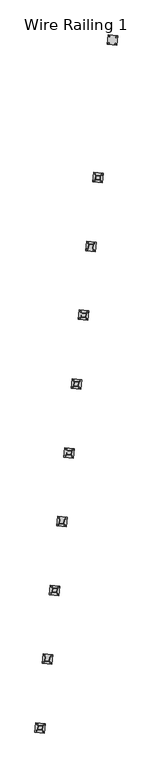
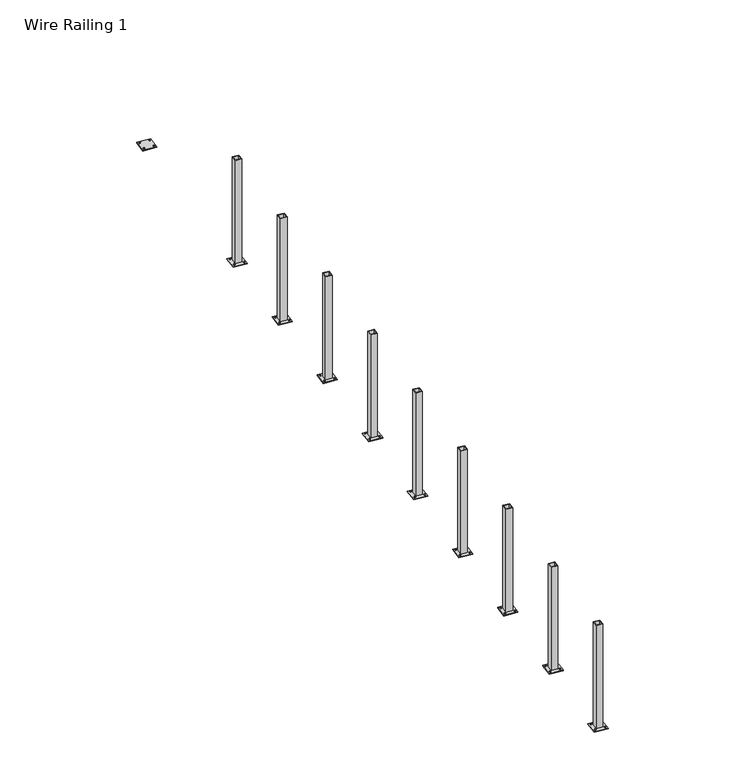
"""IFC4 building model written with IfcOpenShell, lengths in millimetres: railing geometry, Wire Railing 1."""

from ifc_helpers import new_model, si_unit, point, frame, frame_2d, origin, place, context, project, spatial, polyline, circle_curve, trimmed, segment, composite_curve, outline, extrude, source, transform, mapped, element, save


def wire_railing_1_54126149(model_context):
    return source(origin(), model_context, "Body", "SweptSolid", [
        extrude(outline(composite_curve([segment(trimmed(circle_curve(frame_2d((35087.2651438, 39002.031004)), 6.35), [point((35080.9499297, 39002.6947597))], [point((35093.5803578, 39001.3672483))], False, "CARTESIAN"), True, "CONTINUOUS"), segment(trimmed(circle_curve(frame_2d((35087.2651438, 39002.031004)), 6.35), [point((35093.5803578, 39001.3672483))], [point((35080.9499297, 39002.6947597))], False, "CARTESIAN"), True, "CONTINUOUS")], self_intersect=False)), frame((0.0, 0.0, 269252.7), z_axis=(0.0, 0.0, 1.0), x_axis=(1.0, 0.0, 0.0)), (0.0, 0.0, 1.0), 12.7),
        extrude(outline(composite_curve([segment(trimmed(circle_curve(frame_2d((35175.6781403, 38992.7384236)), 6.35), [point((35169.3629262, 38993.4021794))], [point((35181.9933543, 38992.0746679))], False, "CARTESIAN"), True, "CONTINUOUS"), segment(trimmed(circle_curve(frame_2d((35175.6781403, 38992.7384236)), 6.35), [point((35181.9933543, 38992.0746679))], [point((35169.3629262, 38993.4021794))], False, "CARTESIAN"), True, "CONTINUOUS")], self_intersect=False)), frame((0.0, 0.0, 269252.7), z_axis=(0.0, 0.0, 1.0), x_axis=(1.0, 0.0, 0.0)), (0.0, 0.0, 1.0), 12.7),
        extrude(outline(composite_curve([segment(trimmed(circle_curve(frame_2d((35096.5577242, 39090.4440005)), 6.35), [point((35090.2425101, 39091.1077562))], [point((35102.8729382, 39089.7802448))], False, "CARTESIAN"), True, "CONTINUOUS"), segment(trimmed(circle_curve(frame_2d((35096.5577242, 39090.4440005)), 6.35), [point((35102.8729382, 39089.7802448))], [point((35090.2425101, 39091.1077562))], False, "CARTESIAN"), True, "CONTINUOUS")], self_intersect=False)), frame((0.0, 0.0, 269252.7), z_axis=(0.0, 0.0, 1.0), x_axis=(1.0, 0.0, 0.0)), (0.0, 0.0, 1.0), 12.7),
        extrude(outline(composite_curve([segment(trimmed(circle_curve(frame_2d((35184.9707207, 39081.1514201)), 6.35), [point((35178.6555066, 39081.8151759))], [point((35191.2859347, 39080.4876644))], False, "CARTESIAN"), True, "CONTINUOUS"), segment(trimmed(circle_curve(frame_2d((35184.9707207, 39081.1514201)), 6.35), [point((35191.2859347, 39080.4876644))], [point((35178.6555066, 39081.8151759))], False, "CARTESIAN"), True, "CONTINUOUS")], self_intersect=False)), frame((0.0, 0.0, 269252.7), z_axis=(0.0, 0.0, 1.0), x_axis=(1.0, 0.0, 0.0)), (0.0, 0.0, 1.0), 12.7),
        extrude(outline(polyline([(35192.6325152, 38971.8015143), (35066.3282344, 38985.0766291), (35079.6033493, 39111.3809098), (35205.90763, 39098.105795), (35192.6325152, 38971.8015143)])), frame((0.0, 0.0, 269252.7), z_axis=(0.0, 0.0, 1.0), x_axis=(1.0, 0.0, 0.0)), (0.0, 0.0, 1.0), 6.35),
        extrude(outline(polyline([(35162.9623591, 39008.4411056), (35102.9678258, 39014.7467852), (35109.2735053, 39074.7413185), (35169.2680387, 39068.4356389), (35162.9623591, 39008.4411056)]), holes=[polyline([(35157.3109008, 39015.4200754), (35162.2890689, 39062.7841807), (35114.9249636, 39067.7623487), (35109.9467956, 39020.3982435), (35157.3109008, 39015.4200754)])]), frame((0.0, 0.0, 269252.7), z_axis=(0.0, 0.0, 1.0), x_axis=(1.0, 0.0, 0.0)), (0.0, 0.0, 1.0), 1047.75),
        extrude(outline(composite_curve([segment(trimmed(circle_curve(frame_2d((34991.3177498, 38089.1525294)), 6.35), [point((34985.0025358, 38089.8162852))], [point((34997.6329638, 38088.4887737))], False, "CARTESIAN"), True, "CONTINUOUS"), segment(trimmed(circle_curve(frame_2d((34991.3177498, 38089.1525294)), 6.35), [point((34997.6329638, 38088.4887737))], [point((34985.0025358, 38089.8162852))], False, "CARTESIAN"), True, "CONTINUOUS")], self_intersect=False)), frame((0.0, 0.0, 269252.7), z_axis=(0.0, 0.0, 1.0), x_axis=(1.0, 0.0, 0.0)), (0.0, 0.0, 1.0), 12.7),
        extrude(outline(composite_curve([segment(trimmed(circle_curve(frame_2d((35079.7307463, 38079.859949)), 6.35), [point((35073.4155323, 38080.5237048))], [point((35086.0459603, 38079.1961933))], False, "CARTESIAN"), True, "CONTINUOUS"), segment(trimmed(circle_curve(frame_2d((35079.7307463, 38079.859949)), 6.35), [point((35086.0459603, 38079.1961933))], [point((35073.4155323, 38080.5237048))], False, "CARTESIAN"), True, "CONTINUOUS")], self_intersect=False)), frame((0.0, 0.0, 269252.7), z_axis=(0.0, 0.0, 1.0), x_axis=(1.0, 0.0, 0.0)), (0.0, 0.0, 1.0), 12.7),
        extrude(outline(composite_curve([segment(trimmed(circle_curve(frame_2d((35000.6103302, 38177.5655259)), 6.35), [point((34994.2951162, 38178.2292817))], [point((35006.9255442, 38176.9017702))], False, "CARTESIAN"), True, "CONTINUOUS"), segment(trimmed(circle_curve(frame_2d((35000.6103302, 38177.5655259)), 6.35), [point((35006.9255442, 38176.9017702))], [point((34994.2951162, 38178.2292817))], False, "CARTESIAN"), True, "CONTINUOUS")], self_intersect=False)), frame((0.0, 0.0, 269252.7), z_axis=(0.0, 0.0, 1.0), x_axis=(1.0, 0.0, 0.0)), (0.0, 0.0, 1.0), 12.7),
        extrude(outline(composite_curve([segment(trimmed(circle_curve(frame_2d((35089.0233267, 38168.2729455)), 6.35), [point((35082.7081127, 38168.9367013))], [point((35095.3385407, 38167.6091898))], False, "CARTESIAN"), True, "CONTINUOUS"), segment(trimmed(circle_curve(frame_2d((35089.0233267, 38168.2729455)), 6.35), [point((35095.3385407, 38167.6091898))], [point((35082.7081127, 38168.9367013))], False, "CARTESIAN"), True, "CONTINUOUS")], self_intersect=False)), frame((0.0, 0.0, 269252.7), z_axis=(0.0, 0.0, 1.0), x_axis=(1.0, 0.0, 0.0)), (0.0, 0.0, 1.0), 12.7),
        extrude(outline(polyline([(35096.6851212, 38058.9230397), (34970.3808405, 38072.1981545), (34983.6559553, 38198.5024353), (35109.960236, 38185.2273204), (35096.6851212, 38058.9230397)])), frame((0.0, 0.0, 269252.7), z_axis=(0.0, 0.0, 1.0), x_axis=(1.0, 0.0, 0.0)), (0.0, 0.0, 1.0), 6.35),
        extrude(outline(polyline([(35067.0149652, 38095.562631), (35007.0204318, 38101.8683106), (35013.3261114, 38161.8628439), (35073.3206447, 38155.5571644), (35067.0149652, 38095.562631)]), holes=[polyline([(35061.3635069, 38102.5416008), (35066.3416749, 38149.9057061), (35018.9775697, 38154.8838741), (35013.9994016, 38107.5197689), (35061.3635069, 38102.5416008)])]), frame((0.0, 0.0, 269252.7), z_axis=(0.0, 0.0, 1.0), x_axis=(1.0, 0.0, 0.0)), (0.0, 0.0, 1.0), 1047.75),
        extrude(outline(composite_curve([segment(trimmed(circle_curve(frame_2d((34895.3703559, 37176.2740549)), 6.35), [point((34889.0551418, 37176.9378106))], [point((34901.6855699, 37175.6102991))], False, "CARTESIAN"), True, "CONTINUOUS"), segment(trimmed(circle_curve(frame_2d((34895.3703559, 37176.2740549)), 6.35), [point((34901.6855699, 37175.6102991))], [point((34889.0551418, 37176.9378106))], False, "CARTESIAN"), True, "CONTINUOUS")], self_intersect=False)), frame((0.0, 0.0, 269252.7), z_axis=(0.0, 0.0, 1.0), x_axis=(1.0, 0.0, 0.0)), (0.0, 0.0, 1.0), 12.7),
        extrude(outline(composite_curve([segment(trimmed(circle_curve(frame_2d((34983.7833524, 37166.9814745)), 6.35), [point((34977.4681383, 37167.6452302))], [point((34990.0985664, 37166.3177187))], False, "CARTESIAN"), True, "CONTINUOUS"), segment(trimmed(circle_curve(frame_2d((34983.7833524, 37166.9814745)), 6.35), [point((34990.0985664, 37166.3177187))], [point((34977.4681383, 37167.6452302))], False, "CARTESIAN"), True, "CONTINUOUS")], self_intersect=False)), frame((0.0, 0.0, 269252.7), z_axis=(0.0, 0.0, 1.0), x_axis=(1.0, 0.0, 0.0)), (0.0, 0.0, 1.0), 12.7),
        extrude(outline(composite_curve([segment(trimmed(circle_curve(frame_2d((34904.6629362, 37264.6870513)), 6.35), [point((34898.3477222, 37265.3508071))], [point((34910.9781503, 37264.0232956))], False, "CARTESIAN"), True, "CONTINUOUS"), segment(trimmed(circle_curve(frame_2d((34904.6629362, 37264.6870513)), 6.35), [point((34910.9781503, 37264.0232956))], [point((34898.3477222, 37265.3508071))], False, "CARTESIAN"), True, "CONTINUOUS")], self_intersect=False)), frame((0.0, 0.0, 269252.7), z_axis=(0.0, 0.0, 1.0), x_axis=(1.0, 0.0, 0.0)), (0.0, 0.0, 1.0), 12.7),
        extrude(outline(composite_curve([segment(trimmed(circle_curve(frame_2d((34993.0759327, 37255.394471)), 6.35), [point((34986.7607187, 37256.0582267))], [point((34999.3911468, 37254.7307152))], False, "CARTESIAN"), True, "CONTINUOUS"), segment(trimmed(circle_curve(frame_2d((34993.0759327, 37255.394471)), 6.35), [point((34999.3911468, 37254.7307152))], [point((34986.7607187, 37256.0582267))], False, "CARTESIAN"), True, "CONTINUOUS")], self_intersect=False)), frame((0.0, 0.0, 269252.7), z_axis=(0.0, 0.0, 1.0), x_axis=(1.0, 0.0, 0.0)), (0.0, 0.0, 1.0), 12.7),
        extrude(outline(polyline([(35000.7377272, 37146.0445651), (34874.4334465, 37159.31968), (34887.7085614, 37285.6239607), (35014.0128421, 37272.3488458), (35000.7377272, 37146.0445651)])), frame((0.0, 0.0, 269252.7), z_axis=(0.0, 0.0, 1.0), x_axis=(1.0, 0.0, 0.0)), (0.0, 0.0, 1.0), 6.35),
        extrude(outline(polyline([(34971.0675712, 37182.6841565), (34911.0730379, 37188.989836), (34917.3787174, 37248.9843694), (34977.3732507, 37242.6786898), (34971.0675712, 37182.6841565)]), holes=[polyline([(34965.4161129, 37189.6631262), (34970.394281, 37237.0272315), (34923.0301757, 37242.0053996), (34918.0520076, 37194.6412943), (34965.4161129, 37189.6631262)])]), frame((0.0, 0.0, 269252.7), z_axis=(0.0, 0.0, 1.0), x_axis=(1.0, 0.0, 0.0)), (0.0, 0.0, 1.0), 1047.75),
        extrude(outline(composite_curve([segment(trimmed(circle_curve(frame_2d((34799.4229619, 36263.3955803)), 6.35), [point((34793.1077479, 36264.059336))], [point((34805.7381759, 36262.7318245))], False, "CARTESIAN"), True, "CONTINUOUS"), segment(trimmed(circle_curve(frame_2d((34799.4229619, 36263.3955803)), 6.35), [point((34805.7381759, 36262.7318245))], [point((34793.1077479, 36264.059336))], False, "CARTESIAN"), True, "CONTINUOUS")], self_intersect=False)), frame((0.0, 0.0, 269252.7), z_axis=(0.0, 0.0, 1.0), x_axis=(1.0, 0.0, 0.0)), (0.0, 0.0, 1.0), 12.7),
        extrude(outline(composite_curve([segment(trimmed(circle_curve(frame_2d((34887.8359584, 36254.1029999)), 6.35), [point((34881.5207444, 36254.7667556))], [point((34894.1511724, 36253.4392442))], False, "CARTESIAN"), True, "CONTINUOUS"), segment(trimmed(circle_curve(frame_2d((34887.8359584, 36254.1029999)), 6.35), [point((34894.1511724, 36253.4392442))], [point((34881.5207444, 36254.7667556))], False, "CARTESIAN"), True, "CONTINUOUS")], self_intersect=False)), frame((0.0, 0.0, 269252.7), z_axis=(0.0, 0.0, 1.0), x_axis=(1.0, 0.0, 0.0)), (0.0, 0.0, 1.0), 12.7),
        extrude(outline(composite_curve([segment(trimmed(circle_curve(frame_2d((34808.7155423, 36351.8085768)), 6.35), [point((34802.4003282, 36352.4723325))], [point((34815.0307563, 36351.144821))], False, "CARTESIAN"), True, "CONTINUOUS"), segment(trimmed(circle_curve(frame_2d((34808.7155423, 36351.8085768)), 6.35), [point((34815.0307563, 36351.144821))], [point((34802.4003282, 36352.4723325))], False, "CARTESIAN"), True, "CONTINUOUS")], self_intersect=False)), frame((0.0, 0.0, 269252.7), z_axis=(0.0, 0.0, 1.0), x_axis=(1.0, 0.0, 0.0)), (0.0, 0.0, 1.0), 12.7),
        extrude(outline(composite_curve([segment(trimmed(circle_curve(frame_2d((34897.1285388, 36342.5159964)), 6.35), [point((34890.8133247, 36343.1797521))], [point((34903.4437528, 36341.8522407))], False, "CARTESIAN"), True, "CONTINUOUS"), segment(trimmed(circle_curve(frame_2d((34897.1285388, 36342.5159964)), 6.35), [point((34903.4437528, 36341.8522407))], [point((34890.8133247, 36343.1797521))], False, "CARTESIAN"), True, "CONTINUOUS")], self_intersect=False)), frame((0.0, 0.0, 269252.7), z_axis=(0.0, 0.0, 1.0), x_axis=(1.0, 0.0, 0.0)), (0.0, 0.0, 1.0), 12.7),
        extrude(outline(polyline([(34904.7903333, 36233.1660906), (34778.4860526, 36246.4412054), (34791.7611674, 36372.7454861), (34918.0654481, 36359.4703713), (34904.7903333, 36233.1660906)])), frame((0.0, 0.0, 269252.7), z_axis=(0.0, 0.0, 1.0), x_axis=(1.0, 0.0, 0.0)), (0.0, 0.0, 1.0), 6.35),
        extrude(outline(polyline([(34875.1201772, 36269.8056819), (34815.1256439, 36276.1113614), (34821.4313234, 36336.1058948), (34881.4258568, 36329.8002152), (34875.1201772, 36269.8056819)]), holes=[polyline([(34869.4687189, 36276.7846517), (34874.446887, 36324.1487569), (34827.0827817, 36329.126925), (34822.1046137, 36281.7628197), (34869.4687189, 36276.7846517)])]), frame((0.0, 0.0, 269252.7), z_axis=(0.0, 0.0, 1.0), x_axis=(1.0, 0.0, 0.0)), (0.0, 0.0, 1.0), 1047.75),
        extrude(outline(composite_curve([segment(trimmed(circle_curve(frame_2d((34703.4755679, 35350.5171057)), 6.35), [point((34697.1603539, 35351.1808614))], [point((34709.790782, 35349.85335))], False, "CARTESIAN"), True, "CONTINUOUS"), segment(trimmed(circle_curve(frame_2d((34703.4755679, 35350.5171057)), 6.35), [point((34709.790782, 35349.85335))], [point((34697.1603539, 35351.1808614))], False, "CARTESIAN"), True, "CONTINUOUS")], self_intersect=False)), frame((0.0, 0.0, 269252.7), z_axis=(0.0, 0.0, 1.0), x_axis=(1.0, 0.0, 0.0)), (0.0, 0.0, 1.0), 12.7),
        extrude(outline(composite_curve([segment(trimmed(circle_curve(frame_2d((34791.8885644, 35341.2245253)), 6.35), [point((34785.5733504, 35341.8882811))], [point((34798.2037785, 35340.5607696))], False, "CARTESIAN"), True, "CONTINUOUS"), segment(trimmed(circle_curve(frame_2d((34791.8885644, 35341.2245253)), 6.35), [point((34798.2037785, 35340.5607696))], [point((34785.5733504, 35341.8882811))], False, "CARTESIAN"), True, "CONTINUOUS")], self_intersect=False)), frame((0.0, 0.0, 269252.7), z_axis=(0.0, 0.0, 1.0), x_axis=(1.0, 0.0, 0.0)), (0.0, 0.0, 1.0), 12.7),
        extrude(outline(composite_curve([segment(trimmed(circle_curve(frame_2d((34712.7681483, 35438.9301022)), 6.35), [point((34706.4529343, 35439.5938579))], [point((34719.0833624, 35438.2663465))], False, "CARTESIAN"), True, "CONTINUOUS"), segment(trimmed(circle_curve(frame_2d((34712.7681483, 35438.9301022)), 6.35), [point((34719.0833624, 35438.2663465))], [point((34706.4529343, 35439.5938579))], False, "CARTESIAN"), True, "CONTINUOUS")], self_intersect=False)), frame((0.0, 0.0, 269252.7), z_axis=(0.0, 0.0, 1.0), x_axis=(1.0, 0.0, 0.0)), (0.0, 0.0, 1.0), 12.7),
        extrude(outline(composite_curve([segment(trimmed(circle_curve(frame_2d((34801.1811448, 35429.6375218)), 6.35), [point((34794.8659308, 35430.3012776))], [point((34807.4963589, 35428.9737661))], False, "CARTESIAN"), True, "CONTINUOUS"), segment(trimmed(circle_curve(frame_2d((34801.1811448, 35429.6375218)), 6.35), [point((34807.4963589, 35428.9737661))], [point((34794.8659308, 35430.3012776))], False, "CARTESIAN"), True, "CONTINUOUS")], self_intersect=False)), frame((0.0, 0.0, 269252.7), z_axis=(0.0, 0.0, 1.0), x_axis=(1.0, 0.0, 0.0)), (0.0, 0.0, 1.0), 12.7),
        extrude(outline(polyline([(34808.8429393, 35320.287616), (34682.5386586, 35333.5627308), (34695.8137734, 35459.8670115), (34822.1180541, 35446.5918967), (34808.8429393, 35320.287616)])), frame((0.0, 0.0, 269252.7), z_axis=(0.0, 0.0, 1.0), x_axis=(1.0, 0.0, 0.0)), (0.0, 0.0, 1.0), 6.35),
        extrude(outline(polyline([(34779.1727833, 35356.9272073), (34719.1782499, 35363.2328869), (34725.4839295, 35423.2274202), (34785.4784628, 35416.9217407), (34779.1727833, 35356.9272073)]), holes=[polyline([(34773.521325, 35363.9061771), (34778.499493, 35411.2702824), (34731.1353878, 35416.2484504), (34726.1572197, 35368.8843452), (34773.521325, 35363.9061771)])]), frame((0.0, 0.0, 269252.7), z_axis=(0.0, 0.0, 1.0), x_axis=(1.0, 0.0, 0.0)), (0.0, 0.0, 1.0), 1047.75),
        extrude(outline(composite_curve([segment(trimmed(circle_curve(frame_2d((34607.528174, 34437.6386311)), 6.35), [point((34601.2129599, 34438.3023869))], [point((34613.843388, 34436.9748754))], False, "CARTESIAN"), True, "CONTINUOUS"), segment(trimmed(circle_curve(frame_2d((34607.528174, 34437.6386311)), 6.35), [point((34613.843388, 34436.9748754))], [point((34601.2129599, 34438.3023869))], False, "CARTESIAN"), True, "CONTINUOUS")], self_intersect=False)), frame((0.0, 0.0, 269252.7), z_axis=(0.0, 0.0, 1.0), x_axis=(1.0, 0.0, 0.0)), (0.0, 0.0, 1.0), 12.7),
        extrude(outline(composite_curve([segment(trimmed(circle_curve(frame_2d((34695.9411705, 34428.3460508)), 6.35), [point((34689.6259564, 34429.0098065))], [point((34702.2563845, 34427.682295))], False, "CARTESIAN"), True, "CONTINUOUS"), segment(trimmed(circle_curve(frame_2d((34695.9411705, 34428.3460508)), 6.35), [point((34702.2563845, 34427.682295))], [point((34689.6259564, 34429.0098065))], False, "CARTESIAN"), True, "CONTINUOUS")], self_intersect=False)), frame((0.0, 0.0, 269252.7), z_axis=(0.0, 0.0, 1.0), x_axis=(1.0, 0.0, 0.0)), (0.0, 0.0, 1.0), 12.7),
        extrude(outline(composite_curve([segment(trimmed(circle_curve(frame_2d((34616.8207544, 34526.0516276)), 6.35), [point((34610.5055403, 34526.7153834))], [point((34623.1359684, 34525.3878719))], False, "CARTESIAN"), True, "CONTINUOUS"), segment(trimmed(circle_curve(frame_2d((34616.8207544, 34526.0516276)), 6.35), [point((34623.1359684, 34525.3878719))], [point((34610.5055403, 34526.7153834))], False, "CARTESIAN"), True, "CONTINUOUS")], self_intersect=False)), frame((0.0, 0.0, 269252.7), z_axis=(0.0, 0.0, 1.0), x_axis=(1.0, 0.0, 0.0)), (0.0, 0.0, 1.0), 12.7),
        extrude(outline(composite_curve([segment(trimmed(circle_curve(frame_2d((34705.2337509, 34516.7590472)), 6.35), [point((34698.9185368, 34517.422803))], [point((34711.5489649, 34516.0952915))], False, "CARTESIAN"), True, "CONTINUOUS"), segment(trimmed(circle_curve(frame_2d((34705.2337509, 34516.7590472)), 6.35), [point((34711.5489649, 34516.0952915))], [point((34698.9185368, 34517.422803))], False, "CARTESIAN"), True, "CONTINUOUS")], self_intersect=False)), frame((0.0, 0.0, 269252.7), z_axis=(0.0, 0.0, 1.0), x_axis=(1.0, 0.0, 0.0)), (0.0, 0.0, 1.0), 12.7),
        extrude(outline(polyline([(34712.8955454, 34407.4091414), (34586.5912646, 34420.6842563), (34599.8663795, 34546.988537), (34726.1706602, 34533.7134221), (34712.8955454, 34407.4091414)])), frame((0.0, 0.0, 269252.7), z_axis=(0.0, 0.0, 1.0), x_axis=(1.0, 0.0, 0.0)), (0.0, 0.0, 1.0), 6.35),
        extrude(outline(polyline([(34683.2253893, 34444.0487328), (34623.230856, 34450.3544123), (34629.5365355, 34510.3489456), (34689.5310689, 34504.0432661), (34683.2253893, 34444.0487328)]), holes=[polyline([(34677.573931, 34451.0277025), (34682.5520991, 34498.3918078), (34635.1879938, 34503.3699759), (34630.2098257, 34456.0058706), (34677.573931, 34451.0277025)])]), frame((0.0, 0.0, 269252.7), z_axis=(0.0, 0.0, 1.0), x_axis=(1.0, 0.0, 0.0)), (0.0, 0.0, 1.0), 1047.75),
        extrude(outline(composite_curve([segment(trimmed(circle_curve(frame_2d((34511.58078, 33524.7601566)), 6.35), [point((34505.265566, 33525.4239123))], [point((34517.895994, 33524.0964008))], False, "CARTESIAN"), True, "CONTINUOUS"), segment(trimmed(circle_curve(frame_2d((34511.58078, 33524.7601566)), 6.35), [point((34517.895994, 33524.0964008))], [point((34505.265566, 33525.4239123))], False, "CARTESIAN"), True, "CONTINUOUS")], self_intersect=False)), frame((0.0, 0.0, 269252.7), z_axis=(0.0, 0.0, 1.0), x_axis=(1.0, 0.0, 0.0)), (0.0, 0.0, 1.0), 12.7),
        extrude(outline(composite_curve([segment(trimmed(circle_curve(frame_2d((34599.9937765, 33515.4675762)), 6.35), [point((34593.6785625, 33516.1313319))], [point((34606.3089905, 33514.8038204))], False, "CARTESIAN"), True, "CONTINUOUS"), segment(trimmed(circle_curve(frame_2d((34599.9937765, 33515.4675762)), 6.35), [point((34606.3089905, 33514.8038204))], [point((34593.6785625, 33516.1313319))], False, "CARTESIAN"), True, "CONTINUOUS")], self_intersect=False)), frame((0.0, 0.0, 269252.7), z_axis=(0.0, 0.0, 1.0), x_axis=(1.0, 0.0, 0.0)), (0.0, 0.0, 1.0), 12.7),
        extrude(outline(composite_curve([segment(trimmed(circle_curve(frame_2d((34520.8733604, 33613.1731531)), 6.35), [point((34514.5581464, 33613.8369088))], [point((34527.1885744, 33612.5093973))], False, "CARTESIAN"), True, "CONTINUOUS"), segment(trimmed(circle_curve(frame_2d((34520.8733604, 33613.1731531)), 6.35), [point((34527.1885744, 33612.5093973))], [point((34514.5581464, 33613.8369088))], False, "CARTESIAN"), True, "CONTINUOUS")], self_intersect=False)), frame((0.0, 0.0, 269252.7), z_axis=(0.0, 0.0, 1.0), x_axis=(1.0, 0.0, 0.0)), (0.0, 0.0, 1.0), 12.7),
        extrude(outline(composite_curve([segment(trimmed(circle_curve(frame_2d((34609.2863569, 33603.8805727)), 6.35), [point((34602.9711429, 33604.5443284))], [point((34615.6015709, 33603.2168169))], False, "CARTESIAN"), True, "CONTINUOUS"), segment(trimmed(circle_curve(frame_2d((34609.2863569, 33603.8805727)), 6.35), [point((34615.6015709, 33603.2168169))], [point((34602.9711429, 33604.5443284))], False, "CARTESIAN"), True, "CONTINUOUS")], self_intersect=False)), frame((0.0, 0.0, 269252.7), z_axis=(0.0, 0.0, 1.0), x_axis=(1.0, 0.0, 0.0)), (0.0, 0.0, 1.0), 12.7),
        extrude(outline(polyline([(34616.9481514, 33494.5306668), (34490.6438707, 33507.8057817), (34503.9189855, 33634.1100624), (34630.2232662, 33620.8349476), (34616.9481514, 33494.5306668)])), frame((0.0, 0.0, 269252.7), z_axis=(0.0, 0.0, 1.0), x_axis=(1.0, 0.0, 0.0)), (0.0, 0.0, 1.0), 6.35),
        extrude(outline(polyline([(34587.2779953, 33531.1702582), (34527.283462, 33537.4759377), (34533.5891416, 33597.4704711), (34593.5836749, 33591.1647915), (34587.2779953, 33531.1702582)]), holes=[polyline([(34581.6265371, 33538.149228), (34586.6047051, 33585.5133332), (34539.2405999, 33590.4915013), (34534.2624318, 33543.127396), (34581.6265371, 33538.149228)])]), frame((0.0, 0.0, 269252.7), z_axis=(0.0, 0.0, 1.0), x_axis=(1.0, 0.0, 0.0)), (0.0, 0.0, 1.0), 1047.75),
        extrude(outline(composite_curve([segment(trimmed(circle_curve(frame_2d((34415.6333861, 32611.881682)), 6.35), [point((34409.318172, 32612.5454377))], [point((34421.9486001, 32611.2179262))], False, "CARTESIAN"), True, "CONTINUOUS"), segment(trimmed(circle_curve(frame_2d((34415.6333861, 32611.881682)), 6.35), [point((34421.9486001, 32611.2179262))], [point((34409.318172, 32612.5454377))], False, "CARTESIAN"), True, "CONTINUOUS")], self_intersect=False)), frame((0.0, 0.0, 269252.7), z_axis=(0.0, 0.0, 1.0), x_axis=(1.0, 0.0, 0.0)), (0.0, 0.0, 1.0), 12.7),
        extrude(outline(composite_curve([segment(trimmed(circle_curve(frame_2d((34504.0463825, 32602.5891016)), 6.35), [point((34497.7311685, 32603.2528573))], [point((34510.3615966, 32601.9253459))], False, "CARTESIAN"), True, "CONTINUOUS"), segment(trimmed(circle_curve(frame_2d((34504.0463825, 32602.5891016)), 6.35), [point((34510.3615966, 32601.9253459))], [point((34497.7311685, 32603.2528573))], False, "CARTESIAN"), True, "CONTINUOUS")], self_intersect=False)), frame((0.0, 0.0, 269252.7), z_axis=(0.0, 0.0, 1.0), x_axis=(1.0, 0.0, 0.0)), (0.0, 0.0, 1.0), 12.7),
        extrude(outline(composite_curve([segment(trimmed(circle_curve(frame_2d((34424.9259664, 32700.2946785)), 6.35), [point((34418.6107524, 32700.9584342))], [point((34431.2411805, 32699.6309227))], False, "CARTESIAN"), True, "CONTINUOUS"), segment(trimmed(circle_curve(frame_2d((34424.9259664, 32700.2946785)), 6.35), [point((34431.2411805, 32699.6309227))], [point((34418.6107524, 32700.9584342))], False, "CARTESIAN"), True, "CONTINUOUS")], self_intersect=False)), frame((0.0, 0.0, 269252.7), z_axis=(0.0, 0.0, 1.0), x_axis=(1.0, 0.0, 0.0)), (0.0, 0.0, 1.0), 12.7),
        extrude(outline(composite_curve([segment(trimmed(circle_curve(frame_2d((34513.3389629, 32691.0020981)), 6.35), [point((34507.0237489, 32691.6658538))], [point((34519.654177, 32690.3383424))], False, "CARTESIAN"), True, "CONTINUOUS"), segment(trimmed(circle_curve(frame_2d((34513.3389629, 32691.0020981)), 6.35), [point((34519.654177, 32690.3383424))], [point((34507.0237489, 32691.6658538))], False, "CARTESIAN"), True, "CONTINUOUS")], self_intersect=False)), frame((0.0, 0.0, 269252.7), z_axis=(0.0, 0.0, 1.0), x_axis=(1.0, 0.0, 0.0)), (0.0, 0.0, 1.0), 12.7),
        extrude(outline(polyline([(34521.0007574, 32581.6521923), (34394.6964767, 32594.9273071), (34407.9715916, 32721.2315878), (34534.2758723, 32707.956473), (34521.0007574, 32581.6521923)])), frame((0.0, 0.0, 269252.7), z_axis=(0.0, 0.0, 1.0), x_axis=(1.0, 0.0, 0.0)), (0.0, 0.0, 1.0), 6.35),
        extrude(outline(polyline([(34491.3306014, 32618.2917836), (34431.3360681, 32624.5974632), (34437.6417476, 32684.5919965), (34497.6362809, 32678.2863169), (34491.3306014, 32618.2917836)]), holes=[polyline([(34485.6791431, 32625.2707534), (34490.6573112, 32672.6348587), (34443.2932059, 32677.6130267), (34438.3150378, 32630.2489214), (34485.6791431, 32625.2707534)])]), frame((0.0, 0.0, 269252.7), z_axis=(0.0, 0.0, 1.0), x_axis=(1.0, 0.0, 0.0)), (0.0, 0.0, 1.0), 1047.75),
        extrude(outline(composite_curve([segment(trimmed(circle_curve(frame_2d((34319.6859921, 31699.0032074)), 6.35), [point((34313.3707781, 31699.6669632))], [point((34326.0012061, 31698.3394517))], False, "CARTESIAN"), True, "CONTINUOUS"), segment(trimmed(circle_curve(frame_2d((34319.6859921, 31699.0032074)), 6.35), [point((34326.0012061, 31698.3394517))], [point((34313.3707781, 31699.6669632))], False, "CARTESIAN"), True, "CONTINUOUS")], self_intersect=False)), frame((0.0, 0.0, 269252.7), z_axis=(0.0, 0.0, 1.0), x_axis=(1.0, 0.0, 0.0)), (0.0, 0.0, 1.0), 12.7),
        extrude(outline(composite_curve([segment(trimmed(circle_curve(frame_2d((34408.0989886, 31689.710627)), 6.35), [point((34401.7837746, 31690.3743828))], [point((34414.4142026, 31689.0468713))], False, "CARTESIAN"), True, "CONTINUOUS"), segment(trimmed(circle_curve(frame_2d((34408.0989886, 31689.710627)), 6.35), [point((34414.4142026, 31689.0468713))], [point((34401.7837746, 31690.3743828))], False, "CARTESIAN"), True, "CONTINUOUS")], self_intersect=False)), frame((0.0, 0.0, 269252.7), z_axis=(0.0, 0.0, 1.0), x_axis=(1.0, 0.0, 0.0)), (0.0, 0.0, 1.0), 12.7),
        extrude(outline(composite_curve([segment(trimmed(circle_curve(frame_2d((34328.9785725, 31787.4162039)), 6.35), [point((34322.6633584, 31788.0799597))], [point((34335.2937865, 31786.7524482))], False, "CARTESIAN"), True, "CONTINUOUS"), segment(trimmed(circle_curve(frame_2d((34328.9785725, 31787.4162039)), 6.35), [point((34335.2937865, 31786.7524482))], [point((34322.6633584, 31788.0799597))], False, "CARTESIAN"), True, "CONTINUOUS")], self_intersect=False)), frame((0.0, 0.0, 269252.7), z_axis=(0.0, 0.0, 1.0), x_axis=(1.0, 0.0, 0.0)), (0.0, 0.0, 1.0), 12.7),
        extrude(outline(composite_curve([segment(trimmed(circle_curve(frame_2d((34417.391569, 31778.1236235)), 6.35), [point((34411.0763549, 31778.7873793))], [point((34423.706783, 31777.4598678))], False, "CARTESIAN"), True, "CONTINUOUS"), segment(trimmed(circle_curve(frame_2d((34417.391569, 31778.1236235)), 6.35), [point((34423.706783, 31777.4598678))], [point((34411.0763549, 31778.7873793))], False, "CARTESIAN"), True, "CONTINUOUS")], self_intersect=False)), frame((0.0, 0.0, 269252.7), z_axis=(0.0, 0.0, 1.0), x_axis=(1.0, 0.0, 0.0)), (0.0, 0.0, 1.0), 12.7),
        extrude(outline(polyline([(34425.0533635, 31668.7737177), (34298.7490828, 31682.0488325), (34312.0241976, 31808.3531132), (34438.3284783, 31795.0779984), (34425.0533635, 31668.7737177)])), frame((0.0, 0.0, 269252.7), z_axis=(0.0, 0.0, 1.0), x_axis=(1.0, 0.0, 0.0)), (0.0, 0.0, 1.0), 6.35),
        extrude(outline(polyline([(34395.3832074, 31705.413309), (34335.3886741, 31711.7189886), (34341.6943536, 31771.7135219), (34401.688887, 31765.4078424), (34395.3832074, 31705.413309)]), holes=[polyline([(34389.7317491, 31712.3922788), (34394.7099172, 31759.7563841), (34347.3458119, 31764.7345521), (34342.3676439, 31717.3704469), (34389.7317491, 31712.3922788)])]), frame((0.0, 0.0, 269252.7), z_axis=(0.0, 0.0, 1.0), x_axis=(1.0, 0.0, 0.0)), (0.0, 0.0, 1.0), 1047.75),
        extrude(outline(composite_curve([segment(trimmed(circle_curve(frame_2d((35279.1599317, 40827.7879531)), 6.35), [point((35272.8447177, 40828.4517089))], [point((35285.4751457, 40827.1241974))], False, "CARTESIAN"), True, "CONTINUOUS"), segment(trimmed(circle_curve(frame_2d((35279.1599317, 40827.7879531)), 6.35), [point((35285.4751457, 40827.1241974))], [point((35272.8447177, 40828.4517089))], False, "CARTESIAN"), True, "CONTINUOUS")], self_intersect=False)), frame((0.0, 0.0, 269252.7), z_axis=(0.0, 0.0, 1.0), x_axis=(1.0, 0.0, 0.0)), (0.0, 0.0, 1.0), 12.7),
        extrude(outline(composite_curve([segment(trimmed(circle_curve(frame_2d((35367.5729282, 40818.4953728)), 6.35), [point((35361.2577142, 40819.1591285))], [point((35373.8881422, 40817.831617))], False, "CARTESIAN"), True, "CONTINUOUS"), segment(trimmed(circle_curve(frame_2d((35367.5729282, 40818.4953728)), 6.35), [point((35373.8881422, 40817.831617))], [point((35361.2577142, 40819.1591285))], False, "CARTESIAN"), True, "CONTINUOUS")], self_intersect=False)), frame((0.0, 0.0, 269252.7), z_axis=(0.0, 0.0, 1.0), x_axis=(1.0, 0.0, 0.0)), (0.0, 0.0, 1.0), 12.7),
        extrude(outline(composite_curve([segment(trimmed(circle_curve(frame_2d((35288.4525121, 40916.2009496)), 6.35), [point((35282.137298, 40916.8647054))], [point((35294.7677261, 40915.5371939))], False, "CARTESIAN"), True, "CONTINUOUS"), segment(trimmed(circle_curve(frame_2d((35288.4525121, 40916.2009496)), 6.35), [point((35294.7677261, 40915.5371939))], [point((35282.137298, 40916.8647054))], False, "CARTESIAN"), True, "CONTINUOUS")], self_intersect=False)), frame((0.0, 0.0, 269252.7), z_axis=(0.0, 0.0, 1.0), x_axis=(1.0, 0.0, 0.0)), (0.0, 0.0, 1.0), 12.7),
        extrude(outline(composite_curve([segment(trimmed(circle_curve(frame_2d((35376.8655086, 40906.9083693)), 6.35), [point((35370.5502945, 40907.572125))], [point((35383.1807226, 40906.2446135))], False, "CARTESIAN"), True, "CONTINUOUS"), segment(trimmed(circle_curve(frame_2d((35376.8655086, 40906.9083693)), 6.35), [point((35383.1807226, 40906.2446135))], [point((35370.5502945, 40907.572125))], False, "CARTESIAN"), True, "CONTINUOUS")], self_intersect=False)), frame((0.0, 0.0, 269252.7), z_axis=(0.0, 0.0, 1.0), x_axis=(1.0, 0.0, 0.0)), (0.0, 0.0, 1.0), 12.7),
        extrude(outline(polyline([(35384.5273031, 40797.5584634), (35258.2230224, 40810.8335783), (35271.4981372, 40937.137859), (35397.8024179, 40923.8627441), (35384.5273031, 40797.5584634)])), frame((0.0, 0.0, 269252.7), z_axis=(0.0, 0.0, 1.0), x_axis=(1.0, 0.0, 0.0)), (0.0, 0.0, 1.0), 6.35),
    ])


if __name__ == "__main__":
    model = new_model("IFC4")
    model_context = context("Model", 3, world=origin())
    ifc_project = project(units=[si_unit("LENGTHUNIT", "METRE", prefix="MILLI")], contexts=[model_context])
    site = spatial("IfcSite", under=ifc_project)
    building = spatial("IfcBuilding", under=site)
    placement = place(None, origin())
    wire_railing_1_shape = wire_railing_1_54126149(model_context)
    element("IfcRailing", 1, ObjectType="Wire Railing 1", at=placement, inside=building, context=model_context, shape_type="MappedRepresentation", body=[
        mapped(wire_railing_1_shape, transform((0.0, 0.0, 0.0), x_axis=(1.0, 0.0, 0.0), y_axis=(0.0, 1.0, 0.0), z_axis=(0.0, 0.0, 1.0))),
    ])
    save(model, "model.ifc")

# Revit data of these elements
# Element 1 (IfcRailing, "Wire Railing 1")
#   Materials on its faces: "WIRE RAILING"
# Materials
#   "WIRE RAILING": class "Metal", colour RGB 244 244 244, transparency 0, Manufacturer = "Kawneer", URL = "http://www.kawneer.com/kawneer/north_america/en/home.asp", Cost = 0
